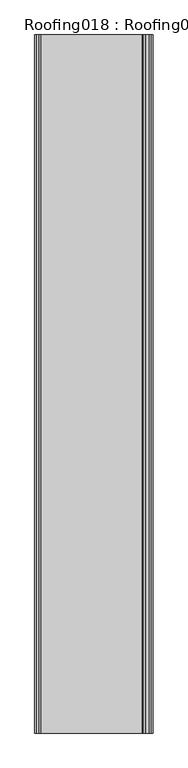
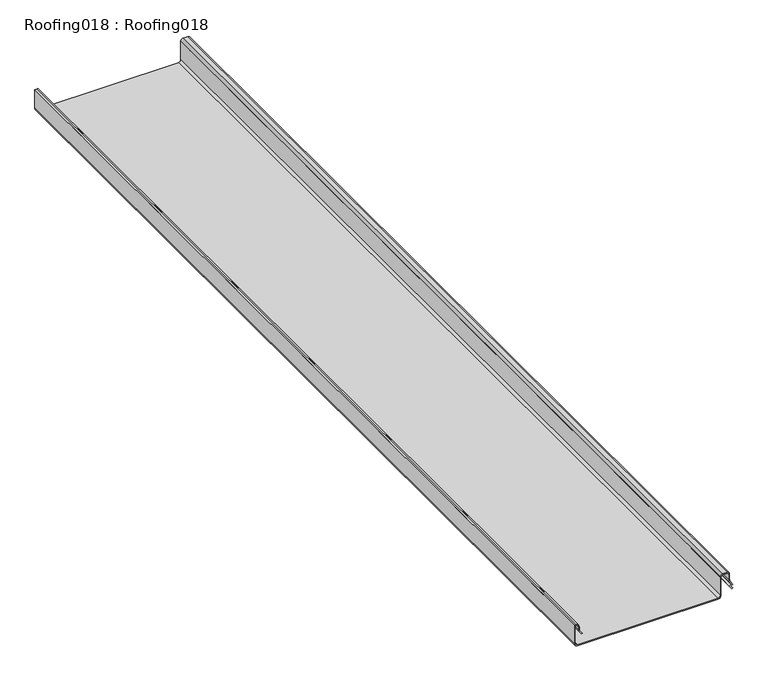
"""IFC4 building model written with IfcOpenShell, lengths in millimetres: proxy geometry, Roofing018 : Roofing018."""

import ifcopenshell
import ifcopenshell.guid

model = None  # the IFC model being written
_history = None  # IfcOwnerHistory: only IFC2X3 demands one
_inside = {}  # id of a spatial element -> (the spatial element, [elements in it])
_under = {}  # id of a project, library or spatial element -> (it, [spatial elements below it])
_declared = {}  # id of a project -> (the project, [libraries it declares])
_typed = {}  # id of a type object -> (the type object, [elements of that type])
_made_of = {}  # id of a material, layer set ... -> (it, [elements and type objects made of it])


def new_model(schema):
    """Start an empty IFC model of exactly this schema.

    Asked for "IFC4X3", IfcOpenShell would pick the latest addendum, in which some entities
    have other attributes; the version numbers below select the first issue.
    IFC2X3 requires an IfcOwnerHistory on every rooted entity: one is made here for all.
    """
    global model, _history
    if schema == "IFC4X3":
        model = ifcopenshell.file(schema_version=(4, 3, 0, 0))
    else:
        model = ifcopenshell.file(schema=schema)
    _inside.clear()
    _under.clear()
    _declared.clear()
    _typed.clear()
    _made_of.clear()
    _history = None
    if model.schema == "IFC2X3":
        org = make("IfcOrganization", Name="unknown")
        user = make(
            "IfcPersonAndOrganization",
            ThePerson=make("IfcPerson", FamilyName="unknown"),
            TheOrganization=org,
        )
        app = make(
            "IfcApplication",
            ApplicationDeveloper=org,
            Version="unknown",
            ApplicationFullName="unknown",
            ApplicationIdentifier="unknown",
        )
        _history = make(
            "IfcOwnerHistory",
            OwningUser=user,
            OwningApplication=app,
            ChangeAction="ADDED",
            CreationDate=0,
        )
    return model


def make(cls, **values):
    """One entity of the class cls with the attributes given. An attribute that is None is left unset."""
    return model.create_entity(
        cls, **{name: value for name, value in values.items() if value is not None}
    )


def rooted(cls, **values):
    """An entity with a GlobalId (a new one), such as an element, a storey or a relation."""
    return make(cls, GlobalId=ifcopenshell.guid.new(), OwnerHistory=_history, **values)


def si_unit(unit_type, name, prefix=None):
    """IfcSIUnit, for example si_unit("LENGTHUNIT", "METRE", prefix="MILLI")."""
    return make("IfcSIUnit", UnitType=unit_type, Prefix=prefix, Name=name)


def assignment(units):
    """IfcUnitAssignment: the units of a project."""
    return None if units is None else make("IfcUnitAssignment", Units=units)


def point(xyz):
    """IfcCartesianPoint."""
    return None if xyz is None else make("IfcCartesianPoint", Coordinates=xyz)


def direction(xyz):
    """IfcDirection."""
    return None if xyz is None else make("IfcDirection", DirectionRatios=xyz)


def frame(location, z_axis=None, x_axis=None):
    """IfcAxis2Placement3D, a coordinate frame: its origin and axes. An axis left out is left unset."""
    return make(
        "IfcAxis2Placement3D",
        Location=point(location),
        Axis=direction(z_axis),
        RefDirection=direction(x_axis),
    )


def frame_2d(location, x_axis=None):
    """IfcAxis2Placement2D, a coordinate frame in the plane: its origin and x axis."""
    return make(
        "IfcAxis2Placement2D", Location=point(location), RefDirection=direction(x_axis)
    )


def origin():
    """The frame at (0, 0, 0) with its axes left unset."""
    return frame((0.0, 0.0, 0.0))


def place(relative_to, where):
    """IfcLocalPlacement: puts the frame where relative to a parent placement (None: the world)."""
    return make(
        "IfcLocalPlacement", PlacementRelTo=relative_to, RelativePlacement=where
    )


def context(
    kind, dimensions, precision=None, world=None, true_north=None, identifier=None
):
    """IfcGeometricRepresentationContext, for example the 3D "Model" context."""
    return make(
        "IfcGeometricRepresentationContext",
        ContextIdentifier=identifier,
        ContextType=kind,
        CoordinateSpaceDimension=dimensions,
        Precision=precision,
        WorldCoordinateSystem=world,
        TrueNorth=true_north,
    )


def project(units=None, contexts=None):
    """IfcProject with its units and contexts."""
    return rooted(
        "IfcProject",
        Name="project",
        RepresentationContexts=contexts,
        UnitsInContext=assignment(units),
    )


def spatial(cls, under=None, at=None, **own):
    """A site, building, storey or space (cls), placed at a placement, below another one or the project."""
    s = rooted(cls, ObjectPlacement=at, **own)
    if under is not None:
        _under.setdefault(under.id(), (under, []))[1].append(s)
    return s


def polyline(points):
    """IfcPolyline through the points."""
    return make("IfcPolyline", Points=[point(p) for p in points])


def circle_curve(where, radius):
    """IfcCircle in the frame where."""
    return make("IfcCircle", Position=where, Radius=radius)


def trimmed(basis, trim1, trim2, sense, master):
    """IfcTrimmedCurve: the piece of a basis curve between two trims."""
    return make(
        "IfcTrimmedCurve",
        BasisCurve=basis,
        Trim1=trim1,
        Trim2=trim2,
        SenseAgreement=sense,
        MasterRepresentation=master,
    )


def segment(curve, same_sense, transition):
    """IfcCompositeCurveSegment."""
    return make(
        "IfcCompositeCurveSegment",
        Transition=transition,
        SameSense=same_sense,
        ParentCurve=curve,
    )


def composite_curve(segments, self_intersect=None):
    """IfcCompositeCurve: segments joined end to end."""
    return make("IfcCompositeCurve", Segments=segments, SelfIntersect=self_intersect)


def outline(outer, holes=None, kind="AREA"):
    """IfcArbitraryClosedProfileDef: a profile drawn as a closed curve; with holes, ...WithVoids."""
    if holes is None:
        return make("IfcArbitraryClosedProfileDef", ProfileType=kind, OuterCurve=outer)
    return make(
        "IfcArbitraryProfileDefWithVoids",
        ProfileType=kind,
        OuterCurve=outer,
        InnerCurves=holes,
    )


def extrude(swept, where, along, depth):
    """IfcExtrudedAreaSolid: the profile swept, set in the frame where, extruded along a direction by depth."""
    return make(
        "IfcExtrudedAreaSolid",
        SweptArea=swept,
        Position=where,
        ExtrudedDirection=direction(along),
        Depth=depth,
    )


def shape(context_of_items, identifier, shape_type, items):
    """IfcShapeRepresentation: the items that make up one representation, for example the "Body"."""
    return make(
        "IfcShapeRepresentation",
        ContextOfItems=context_of_items,
        RepresentationIdentifier=identifier,
        RepresentationType=shape_type,
        Items=items,
    )


def source(mapping_origin, context_of_items, identifier, shape_type, items):
    """IfcRepresentationMap: a shape defined once, which mapped items show again and again."""
    return make(
        "IfcRepresentationMap",
        MappingOrigin=mapping_origin,
        MappedRepresentation=shape(context_of_items, identifier, shape_type, items),
    )


def transform(
    local_origin,
    x_axis=None,
    y_axis=None,
    z_axis=None,
    scale=None,
    scale2=None,
    scale3=None,
    uniform=True,
):
    """IfcCartesianTransformationOperator3D, or its non-uniform kind. x_axis, y_axis, z_axis: its Axis1, 2, 3."""
    if uniform:
        return make(
            "IfcCartesianTransformationOperator3D",
            Axis1=direction(x_axis),
            Axis2=direction(y_axis),
            LocalOrigin=point(local_origin),
            Scale=scale,
            Axis3=direction(z_axis),
        )
    return make(
        "IfcCartesianTransformationOperator3DnonUniform",
        Axis1=direction(x_axis),
        Axis2=direction(y_axis),
        LocalOrigin=point(local_origin),
        Scale=scale,
        Axis3=direction(z_axis),
        Scale2=scale2,
        Scale3=scale3,
    )


def mapped(mapping_source, mapping_target):
    """IfcMappedItem: shows the shape of a source again, moved by a transform."""
    return make(
        "IfcMappedItem", MappingSource=mapping_source, MappingTarget=mapping_target
    )


def made_of(thing, what):
    """Note that an element or type object is made of a material, layer set ...; save() writes the relation."""
    if what is not None:
        _made_of.setdefault(what.id(), (what, []))[1].append(thing)
    return thing


def element(
    cls,
    number,
    at=None,
    inside=None,
    cuts=None,
    type_object=None,
    material=None,
    context=None,
    identifier="Body",
    shape_type=None,
    held_by="IfcProductDefinitionShape",
    body=None,
    shapes=None,
    **own,
):
    """One element of the class cls, such as IfcWall. Its Tag is "e" and its number.

    at: its placement. inside: the storey or other place that contains it. cuts: it is an
    opening in that element (IfcRelVoidsElement). A single representation is given by context,
    identifier, shape_type and body (its items); several are given by shapes. held_by: the class
    of the entity that holds the representations. save() writes the other relations.
    """
    e = rooted(cls, Tag="e%d" % number, ObjectPlacement=at, **own)
    if body is not None:
        shapes = [shape(context, identifier, shape_type, body)]
    if shapes is not None:
        e.Representation = make(held_by, Representations=shapes)
    if inside is not None:
        _inside.setdefault(inside.id(), (inside, []))[1].append(e)
    if cuts is not None:
        rooted(
            "IfcRelVoidsElement", RelatingBuildingElement=cuts, RelatedOpeningElement=e
        )
    if type_object is not None:
        _typed.setdefault(type_object.id(), (type_object, []))[1].append(e)
    return made_of(e, material)


def aggregate(whole, parts):
    """IfcRelAggregates: a whole, such as a stair, and the parts it consists of."""
    return rooted("IfcRelAggregates", RelatingObject=whole, RelatedObjects=parts)


def save(model, path):
    """Write the relations noted so far, then the file.

    IfcRelAggregates (storeys below a building ...), IfcRelContainedInSpatialStructure (elements
    in a storey), IfcRelDefinesByType, IfcRelAssociatesMaterial and IfcRelDeclares: one each for
    every whole, place, type object, material and project.
    """
    for whole, parts in _under.values():
        aggregate(whole, parts)
    for where, things in _inside.values():
        rooted(
            "IfcRelContainedInSpatialStructure",
            RelatedElements=things,
            RelatingStructure=where,
        )
    for kind, things in _typed.values():
        rooted("IfcRelDefinesByType", RelatedObjects=things, RelatingType=kind)
    for what, things in _made_of.values():
        rooted("IfcRelAssociatesMaterial", RelatedObjects=things, RelatingMaterial=what)
    for by, libraries in _declared.values():
        rooted("IfcRelDeclares", RelatingContext=by, RelatedDefinitions=libraries)
    model.write(path)


def roofing018_roofing018_b64cce71(model_context):
    return source(origin(), model_context, "Body", "SweptSolid", [
        extrude(outline(composite_curve([segment(polyline([(41810.80004, 5193.0168476), (41802.3258778, 5199.1644962), (41803.5002989, 5200.7833647), (41811.974461, 5194.6357161)]), True, "CONTINUOUS"), segment(trimmed(circle_curve(frame_2d((41813.7830695, 5197.1287736)), 3.08), [point((41811.974461, 5194.6357161))], [point((41813.7830695, 5194.0487736))], True, "CARTESIAN"), True, "CONTINUOUS"), segment(polyline([(41813.7830695, 5194.0487736), (41820.5396278, 5194.0487736)]), True, "CONTINUOUS"), segment(trimmed(circle_curve(frame_2d((41820.5396278, 5186.9687736)), 7.08), [point((41820.5396278, 5194.0487736))], [point((41827.6196278, 5186.9687736))], False, "CARTESIAN"), True, "CONTINUOUS"), segment(polyline([(41827.6196278, 5186.9687736), (41827.6196278, 5183.3739689), (41785.8824403, 5183.3739689)]), True, "CONTINUOUS"), segment(trimmed(circle_curve(frame_2d((41785.8824403, 5190.4539689)), 7.08), [point((41785.8824403, 5183.3739689))], [point((41778.8024403, 5190.4539689))], False, "CARTESIAN"), True, "CONTINUOUS"), segment(polyline([(41778.8024403, 5190.4539689), (41778.8024403, 5490.7280509)]), True, "CONTINUOUS"), segment(trimmed(circle_curve(frame_2d((41785.8824403, 5490.7280509)), 7.08), [point((41778.8024403, 5490.7280509))], [point((41785.8824403, 5497.8080509))], False, "CARTESIAN"), True, "CONTINUOUS"), segment(polyline([(41785.8824403, 5497.8080509), (41827.4958778, 5497.8080509)]), True, "CONTINUOUS"), segment(trimmed(circle_curve(frame_2d((41827.4958778, 5500.8880509)), 3.08), [point((41827.4958778, 5497.8080509))], [point((41830.5758778, 5500.8880509))], True, "CARTESIAN"), True, "CONTINUOUS"), segment(polyline([(41830.5758778, 5500.8880509), (41830.5758778, 5510.8958278)]), True, "CONTINUOUS"), segment(trimmed(circle_curve(frame_2d((41827.4958778, 5510.8958278)), 3.08), [point((41830.5758778, 5510.8958278))], [point((41827.4958778, 5513.9758278))], True, "CARTESIAN"), True, "CONTINUOUS"), segment(polyline([(41827.4958778, 5513.9758278), (41814.3133037, 5513.9758278)]), True, "CONTINUOUS"), segment(trimmed(circle_curve(frame_2d((41814.3133037, 5521.0558278)), 7.08), [point((41814.3133037, 5513.9758278))], [point((41810.8234609, 5514.8956819))], False, "CARTESIAN"), True, "CONTINUOUS"), segment(polyline([(41810.8234609, 5514.8956819), (41801.98033, 5519.9054879), (41799.4289318, 5515.5538231), (41792.0466166, 5520.8241475), (41793.2086903, 5522.451902), (41798.8102528, 5518.4528786), (41801.2516591, 5522.6169411), (41811.8092922, 5516.6358361)]), True, "CONTINUOUS"), segment(trimmed(circle_curve(frame_2d((41814.3133037, 5521.0558278)), 5.08), [point((41811.8092922, 5516.6358361))], [point((41814.3133037, 5515.9758278))], True, "CARTESIAN"), True, "CONTINUOUS"), segment(polyline([(41814.3133037, 5515.9758278), (41827.4958778, 5515.9758278)]), True, "CONTINUOUS"), segment(trimmed(circle_curve(frame_2d((41827.4958778, 5510.8958278)), 5.08), [point((41827.4958778, 5515.9758278))], [point((41832.5758778, 5510.8958278))], False, "CARTESIAN"), True, "CONTINUOUS"), segment(polyline([(41832.5758778, 5510.8958278), (41832.5758778, 5500.8880509)]), True, "CONTINUOUS"), segment(trimmed(circle_curve(frame_2d((41827.4958778, 5500.8880509)), 5.08), [point((41832.5758778, 5500.8880509))], [point((41827.4958778, 5495.8080509))], False, "CARTESIAN"), True, "CONTINUOUS"), segment(polyline([(41827.4958778, 5495.8080509), (41785.8824403, 5495.8080509)]), True, "CONTINUOUS"), segment(trimmed(circle_curve(frame_2d((41785.8824403, 5490.7280509)), 5.08), [point((41785.8824403, 5495.8080509))], [point((41780.8024403, 5490.7280509))], True, "CARTESIAN"), True, "CONTINUOUS"), segment(polyline([(41780.8024403, 5490.7280509), (41780.8024403, 5190.4539689)]), True, "CONTINUOUS"), segment(trimmed(circle_curve(frame_2d((41785.8824403, 5190.4539689)), 5.08), [point((41780.8024403, 5190.4539689))], [point((41785.8824403, 5185.3739689))], True, "CARTESIAN"), True, "CONTINUOUS"), segment(polyline([(41785.8824403, 5185.3739689), (41825.6196278, 5185.3739689), (41825.6196278, 5186.9687736)]), True, "CONTINUOUS"), segment(trimmed(circle_curve(frame_2d((41820.5396278, 5186.9687736)), 5.08), [point((41825.6196278, 5186.9687736))], [point((41820.5396278, 5192.0487736))], True, "CARTESIAN"), True, "CONTINUOUS"), segment(polyline([(41820.5396278, 5192.0487736), (41813.7830695, 5192.0487736)]), True, "CONTINUOUS"), segment(trimmed(circle_curve(frame_2d((41813.7830695, 5197.1287736)), 5.08), [point((41813.7830695, 5192.0487736))], [point((41810.80004, 5193.0168476))], False, "CARTESIAN"), True, "CONTINUOUS")], self_intersect=False)), frame((0.0, 2217.3609988, 0.0), z_axis=(0.0, 1.0, 0.0), x_axis=(0.0, 0.0, 1.0)), (0.0, 0.0, 1.0), 2000.0),
    ])


if __name__ == "__main__":
    model = new_model("IFC4")
    model_context = context("Model", 3, world=origin())
    ifc_project = project(units=[si_unit("LENGTHUNIT", "METRE", prefix="MILLI")], contexts=[model_context])
    site = spatial("IfcSite", under=ifc_project)
    building = spatial("IfcBuilding", under=site)
    placement = place(None, origin())
    roofing018_roofing018_shape = roofing018_roofing018_b64cce71(model_context)
    element("IfcBuildingElementProxy", 1, Name="Roofing018 : Roofing018", ObjectType="Roofing018 : Roofing018", at=placement, inside=building, context=model_context, shape_type="MappedRepresentation", body=[
        mapped(roofing018_roofing018_shape, transform((0.0, 0.0, 0.0), x_axis=(1.0, 0.0, 0.0), y_axis=(0.0, 1.0, 0.0), z_axis=(0.0, 0.0, 1.0))),
    ])
    save(model, "model.ifc")

# Revit data of these elements
# Type "Roofing018 : Roofing018"
#   NameOverride = "Roofing018"
# Element 1 (IfcBuildingElementProxy, "Roofing018 : Roofing018")
#   Materials on its faces: "STANDING SEAM METAL ROOF FOLLOW MANU. RECOMMENDED EDGE/TRANSITION DETAILS"
# Materials
#   "STANDING SEAM METAL ROOF FOLLOW MANU. RECOMMENDED EDGE/TRANSITION DETAILS": class "Unassigned", colour RGB 128 128 128, transparency 0, Cost = 0
